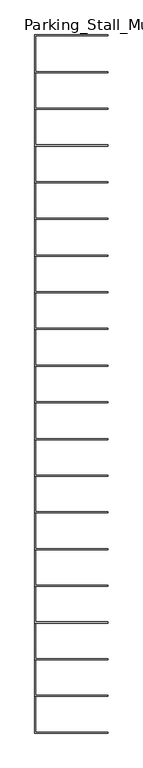
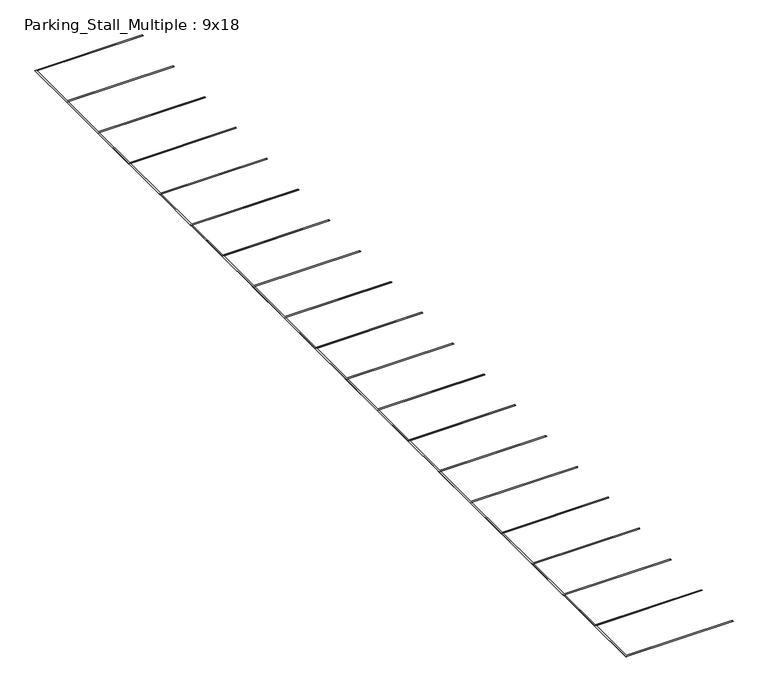
"""IFC4 building model written with IfcOpenShell, lengths in millimetres: proxy geometry, Parking_Stall_Multiple : 9x18."""

from ifc_helpers import new_model, si_unit, origin, origin_with_axes, place, context, project, spatial, polyline, outline, extrude, source, transform, mapped, element, save


def parking_stall_multiple_9x18_bfa5105c(model_context):
    return source(origin(), model_context, "Body", "SweptSolid", [
        extrude(outline(polyline([(5486.4, 49377.6), (0.0, 49377.6), (0.0, 52197.0), (5486.4, 52197.0), (5486.4, 52120.8), (76.2, 52120.8), (76.2, 49453.8), (5486.4, 49453.8), (5486.4, 49377.6)])), origin_with_axes(), (0.0, 0.0, 1.0), 6.35),
        extrude(outline(polyline([(5486.4, 46634.4), (0.0, 46634.4), (0.0, 49453.8), (5486.4, 49453.8), (5486.4, 49377.6), (76.2, 49377.6), (76.2, 46710.6), (5486.4, 46710.6), (5486.4, 46634.4)])), origin_with_axes(), (0.0, 0.0, 1.0), 6.35),
        extrude(outline(polyline([(5486.4, 43891.2), (0.0, 43891.2), (0.0, 46710.6), (5486.4, 46710.6), (5486.4, 46634.4), (76.2, 46634.4), (76.2, 43967.4), (5486.4, 43967.4), (5486.4, 43891.2)])), origin_with_axes(), (0.0, 0.0, 1.0), 6.35),
        extrude(outline(polyline([(5486.4, 41148.0), (0.0, 41148.0), (0.0, 43967.4), (5486.4, 43967.4), (5486.4, 43891.2), (76.2, 43891.2), (76.2, 41224.2), (5486.4, 41224.2), (5486.4, 41148.0)])), origin_with_axes(), (0.0, 0.0, 1.0), 6.35),
        extrude(outline(polyline([(5486.4, 38404.8), (0.0, 38404.8), (0.0, 41224.2), (5486.4, 41224.2), (5486.4, 41148.0), (76.2, 41148.0), (76.2, 38481.0), (5486.4, 38481.0), (5486.4, 38404.8)])), origin_with_axes(), (0.0, 0.0, 1.0), 6.35),
        extrude(outline(polyline([(5486.4, 35661.6), (0.0, 35661.6), (0.0, 38481.0), (5486.4, 38481.0), (5486.4, 38404.8), (76.2, 38404.8), (76.2, 35737.8), (5486.4, 35737.8), (5486.4, 35661.6)])), origin_with_axes(), (0.0, 0.0, 1.0), 6.35),
        extrude(outline(polyline([(5486.4, 32918.4), (0.0, 32918.4), (0.0, 35737.8), (5486.4, 35737.8), (5486.4, 35661.6), (76.2, 35661.6), (76.2, 32994.6), (5486.4, 32994.6), (5486.4, 32918.4)])), origin_with_axes(), (0.0, 0.0, 1.0), 6.35),
        extrude(outline(polyline([(5486.4, 30175.2), (0.0, 30175.2), (0.0, 32994.6), (5486.4, 32994.6), (5486.4, 32918.4), (76.2, 32918.4), (76.2, 30251.4), (5486.4, 30251.4), (5486.4, 30175.2)])), origin_with_axes(), (0.0, 0.0, 1.0), 6.35),
        extrude(outline(polyline([(5486.4, 27432.0), (0.0, 27432.0), (0.0, 30251.4), (5486.4, 30251.4), (5486.4, 30175.2), (76.2, 30175.2), (76.2, 27508.2), (5486.4, 27508.2), (5486.4, 27432.0)])), origin_with_axes(), (0.0, 0.0, 1.0), 6.35),
        extrude(outline(polyline([(5486.4, 24688.8), (0.0, 24688.8), (0.0, 27508.2), (5486.4, 27508.2), (5486.4, 27432.0), (76.2, 27432.0), (76.2, 24765.0), (5486.4, 24765.0), (5486.4, 24688.8)])), origin_with_axes(), (0.0, 0.0, 1.0), 6.35),
        extrude(outline(polyline([(5486.4, 21945.6), (0.0, 21945.6), (0.0, 24765.0), (5486.4, 24765.0), (5486.4, 24688.8), (76.2, 24688.8), (76.2, 22021.8), (5486.4, 22021.8), (5486.4, 21945.6)])), origin_with_axes(), (0.0, 0.0, 1.0), 6.35),
        extrude(outline(polyline([(5486.4, 19202.4), (0.0, 19202.4), (0.0, 22021.8), (5486.4, 22021.8), (5486.4, 21945.6), (76.2, 21945.6), (76.2, 19278.6), (5486.4, 19278.6), (5486.4, 19202.4)])), origin_with_axes(), (0.0, 0.0, 1.0), 6.35),
        extrude(outline(polyline([(5486.4, 16459.2), (0.0, 16459.2), (0.0, 19278.6), (5486.4, 19278.6), (5486.4, 19202.4), (76.2, 19202.4), (76.2, 16535.4), (5486.4, 16535.4), (5486.4, 16459.2)])), origin_with_axes(), (0.0, 0.0, 1.0), 6.35),
        extrude(outline(polyline([(5486.4, 13716.0), (0.0, 13716.0), (0.0, 16535.4), (5486.4, 16535.4), (5486.4, 16459.2), (76.2, 16459.2), (76.2, 13792.2), (5486.4, 13792.2), (5486.4, 13716.0)])), origin_with_axes(), (0.0, 0.0, 1.0), 6.35),
        extrude(outline(polyline([(5486.4, 10972.8), (0.0, 10972.8), (0.0, 13792.2), (5486.4, 13792.2), (5486.4, 13716.0), (76.2, 13716.0), (76.2, 11049.0), (5486.4, 11049.0), (5486.4, 10972.8)])), origin_with_axes(), (0.0, 0.0, 1.0), 6.35),
        extrude(outline(polyline([(5486.4, 8229.6), (0.0, 8229.6), (0.0, 11049.0), (5486.4, 11049.0), (5486.4, 10972.8), (76.2, 10972.8), (76.2, 8305.8), (5486.4, 8305.8), (5486.4, 8229.6)])), origin_with_axes(), (0.0, 0.0, 1.0), 6.35),
        extrude(outline(polyline([(5486.4, 5486.4), (0.0, 5486.4), (0.0, 8305.8), (5486.4, 8305.8), (5486.4, 8229.6), (76.2, 8229.6), (76.2, 5562.6), (5486.4, 5562.6), (5486.4, 5486.4)])), origin_with_axes(), (0.0, 0.0, 1.0), 6.35),
        extrude(outline(polyline([(5486.4, 2743.2), (0.0, 2743.2), (0.0, 5562.6), (5486.4, 5562.6), (5486.4, 5486.4), (76.2, 5486.4), (76.2, 2819.4), (5486.4, 2819.4), (5486.4, 2743.2)])), origin_with_axes(), (0.0, 0.0, 1.0), 6.35),
        extrude(outline(polyline([(5486.4, 0.0), (0.0, 0.0), (0.0, 2819.4), (5486.4, 2819.4), (5486.4, 2743.2), (76.2, 2743.2), (76.2, 76.2), (5486.4, 76.2), (5486.4, 0.0)])), origin_with_axes(), (0.0, 0.0, 1.0), 6.35),
    ])


if __name__ == "__main__":
    model = new_model("IFC4")
    model_context = context("Model", 3, world=origin())
    ifc_project = project(units=[si_unit("LENGTHUNIT", "METRE", prefix="MILLI")], contexts=[model_context])
    site = spatial("IfcSite", under=ifc_project)
    building = spatial("IfcBuilding", under=site)
    placement = place(None, origin())
    parking_stall_multiple_9x18_shape = parking_stall_multiple_9x18_bfa5105c(model_context)
    element("IfcBuildingElementProxy", 1, Name="Parking_Stall_Multiple : 9x18", ObjectType="Parking_Stall_Multiple : 9x18", at=placement, inside=building, context=model_context, shape_type="MappedRepresentation", body=[
        mapped(parking_stall_multiple_9x18_shape, transform((0.0, 0.0, 0.0), x_axis=(1.0, 0.0, 0.0), y_axis=(0.0, 1.0, 0.0), z_axis=(0.0, 0.0, 1.0))),
    ])
    save(model, "model.ifc")

# Revit data of these elements
# Type "Parking_Stall_Multiple : 9x18"
#   Parking_Width_M = 9' - 0"
#   Parking_Run_Length [instance default] = 65' - 0"
#   Parking_Line_Width = 0' - 3"
#   Parking_Length_M = 18' - 0"
#   Single_Parking_Visibility [instance default] = no
#   Parking_ADA_Symbol = no
#   ParkingUnitsArray [instance default] = 7
#   ParkingUnits [instance default] = 7
#   Multiple_Parking_Visibility [instance default] = yes
#   Parking_Line_Material = none
# Element 1 (IfcBuildingElementProxy, "Parking_Stall_Multiple : 9x18")
#   Parking_Run_Length = 171' - 6.01339"
#   ParkingUnitsArray = 19
#   ParkingUnits = 19
